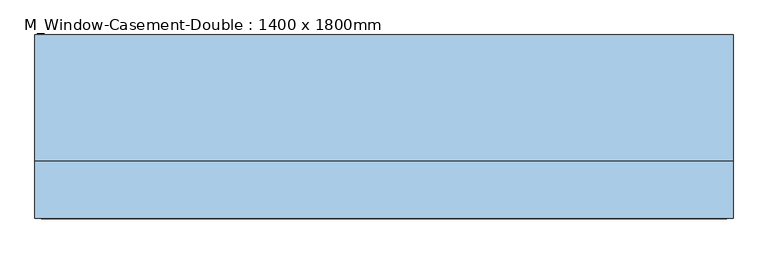
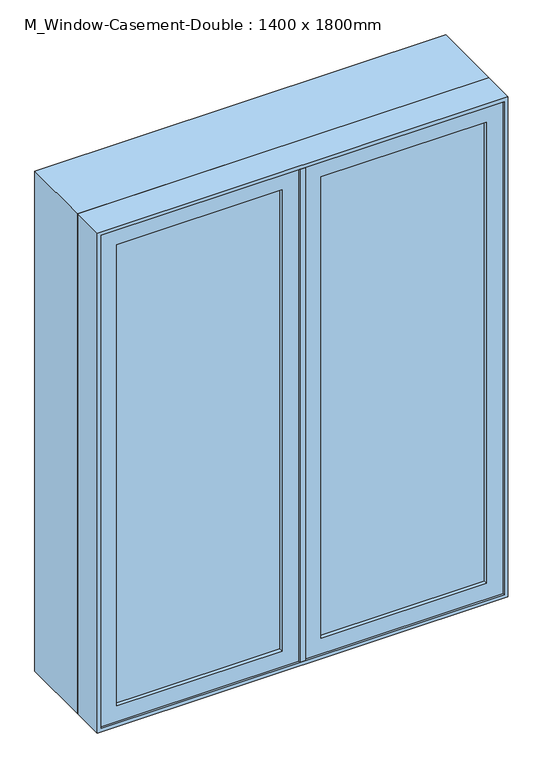
"""IFC4 building model written with IfcOpenShell, lengths in millimetres: window geometry, M_Window-Casement-Double : 1400 x 1800mm."""

import ifcopenshell
import ifcopenshell.guid

model = None  # the IFC model being written
_history = None  # IfcOwnerHistory: only IFC2X3 demands one
_inside = {}  # id of a spatial element -> (the spatial element, [elements in it])
_under = {}  # id of a project, library or spatial element -> (it, [spatial elements below it])
_declared = {}  # id of a project -> (the project, [libraries it declares])
_typed = {}  # id of a type object -> (the type object, [elements of that type])
_made_of = {}  # id of a material, layer set ... -> (it, [elements and type objects made of it])


def new_model(schema):
    """Start an empty IFC model of exactly this schema.

    Asked for "IFC4X3", IfcOpenShell would pick the latest addendum, in which some entities
    have other attributes; the version numbers below select the first issue.
    IFC2X3 requires an IfcOwnerHistory on every rooted entity: one is made here for all.
    """
    global model, _history
    if schema == "IFC4X3":
        model = ifcopenshell.file(schema_version=(4, 3, 0, 0))
    else:
        model = ifcopenshell.file(schema=schema)
    _inside.clear()
    _under.clear()
    _declared.clear()
    _typed.clear()
    _made_of.clear()
    _history = None
    if model.schema == "IFC2X3":
        org = make("IfcOrganization", Name="unknown")
        user = make(
            "IfcPersonAndOrganization",
            ThePerson=make("IfcPerson", FamilyName="unknown"),
            TheOrganization=org,
        )
        app = make(
            "IfcApplication",
            ApplicationDeveloper=org,
            Version="unknown",
            ApplicationFullName="unknown",
            ApplicationIdentifier="unknown",
        )
        _history = make(
            "IfcOwnerHistory",
            OwningUser=user,
            OwningApplication=app,
            ChangeAction="ADDED",
            CreationDate=0,
        )
    return model


def make(cls, **values):
    """One entity of the class cls with the attributes given. An attribute that is None is left unset."""
    return model.create_entity(
        cls, **{name: value for name, value in values.items() if value is not None}
    )


def rooted(cls, **values):
    """An entity with a GlobalId (a new one), such as an element, a storey or a relation."""
    return make(cls, GlobalId=ifcopenshell.guid.new(), OwnerHistory=_history, **values)


def si_unit(unit_type, name, prefix=None):
    """IfcSIUnit, for example si_unit("LENGTHUNIT", "METRE", prefix="MILLI")."""
    return make("IfcSIUnit", UnitType=unit_type, Prefix=prefix, Name=name)


def assignment(units):
    """IfcUnitAssignment: the units of a project."""
    return None if units is None else make("IfcUnitAssignment", Units=units)


def point(xyz):
    """IfcCartesianPoint."""
    return None if xyz is None else make("IfcCartesianPoint", Coordinates=xyz)


def direction(xyz):
    """IfcDirection."""
    return None if xyz is None else make("IfcDirection", DirectionRatios=xyz)


def frame(location, z_axis=None, x_axis=None):
    """IfcAxis2Placement3D, a coordinate frame: its origin and axes. An axis left out is left unset."""
    return make(
        "IfcAxis2Placement3D",
        Location=point(location),
        Axis=direction(z_axis),
        RefDirection=direction(x_axis),
    )


def origin():
    """The frame at (0, 0, 0) with its axes left unset."""
    return frame((0.0, 0.0, 0.0))


def place(relative_to, where):
    """IfcLocalPlacement: puts the frame where relative to a parent placement (None: the world)."""
    return make(
        "IfcLocalPlacement", PlacementRelTo=relative_to, RelativePlacement=where
    )


def context(
    kind, dimensions, precision=None, world=None, true_north=None, identifier=None
):
    """IfcGeometricRepresentationContext, for example the 3D "Model" context."""
    return make(
        "IfcGeometricRepresentationContext",
        ContextIdentifier=identifier,
        ContextType=kind,
        CoordinateSpaceDimension=dimensions,
        Precision=precision,
        WorldCoordinateSystem=world,
        TrueNorth=true_north,
    )


def project(units=None, contexts=None):
    """IfcProject with its units and contexts."""
    return rooted(
        "IfcProject",
        Name="project",
        RepresentationContexts=contexts,
        UnitsInContext=assignment(units),
    )


def spatial(cls, under=None, at=None, **own):
    """A site, building, storey or space (cls), placed at a placement, below another one or the project."""
    s = rooted(cls, ObjectPlacement=at, **own)
    if under is not None:
        _under.setdefault(under.id(), (under, []))[1].append(s)
    return s


def polyline(points):
    """IfcPolyline through the points."""
    return make("IfcPolyline", Points=[point(p) for p in points])


def outline(outer, holes=None, kind="AREA"):
    """IfcArbitraryClosedProfileDef: a profile drawn as a closed curve; with holes, ...WithVoids."""
    if holes is None:
        return make("IfcArbitraryClosedProfileDef", ProfileType=kind, OuterCurve=outer)
    return make(
        "IfcArbitraryProfileDefWithVoids",
        ProfileType=kind,
        OuterCurve=outer,
        InnerCurves=holes,
    )


def extrude(swept, where, along, depth):
    """IfcExtrudedAreaSolid: the profile swept, set in the frame where, extruded along a direction by depth."""
    return make(
        "IfcExtrudedAreaSolid",
        SweptArea=swept,
        Position=where,
        ExtrudedDirection=direction(along),
        Depth=depth,
    )


def faces_of(points, faces, orient=None, outer=None):
    """IfcFace entities. A face is a list of loops; a loop is a list of indices into points, from 0.

    orient and outer hold one flag for each loop. By default every Orientation is true, the
    first loop of a face is its IfcFaceOuterBound and the others are IfcFaceBound.
    """
    made = []
    for i, loops in enumerate(faces):
        bounds = []
        for j, loop in enumerate(loops):
            is_outer = j == 0 if outer is None else outer[i][j]
            bounds.append(
                make(
                    "IfcFaceOuterBound" if is_outer else "IfcFaceBound",
                    Bound=make("IfcPolyLoop", Polygon=[points[k] for k in loop]),
                    Orientation=True if orient is None else orient[i][j],
                )
            )
        made.append(make("IfcFace", Bounds=bounds))
    return made


def faceted_brep(points, faces, orient=None, outer=None, voids=None):
    """IfcFacetedBrep: a solid bounded by flat faces; with voids (closed shells), ...WithVoids."""
    shared = [point(p) for p in points]
    hull = make("IfcClosedShell", CfsFaces=faces_of(shared, faces, orient, outer))
    if voids is None:
        return make("IfcFacetedBrep", Outer=hull)
    return make(
        "IfcFacetedBrepWithVoids",
        Outer=hull,
        Voids=[
            make(cls, CfsFaces=faces_of(shared, fs, o, b)) for cls, fs, o, b in voids
        ],
    )


def shape(context_of_items, identifier, shape_type, items):
    """IfcShapeRepresentation: the items that make up one representation, for example the "Body"."""
    return make(
        "IfcShapeRepresentation",
        ContextOfItems=context_of_items,
        RepresentationIdentifier=identifier,
        RepresentationType=shape_type,
        Items=items,
    )


def source(mapping_origin, context_of_items, identifier, shape_type, items):
    """IfcRepresentationMap: a shape defined once, which mapped items show again and again."""
    return make(
        "IfcRepresentationMap",
        MappingOrigin=mapping_origin,
        MappedRepresentation=shape(context_of_items, identifier, shape_type, items),
    )


def transform(
    local_origin,
    x_axis=None,
    y_axis=None,
    z_axis=None,
    scale=None,
    scale2=None,
    scale3=None,
    uniform=True,
):
    """IfcCartesianTransformationOperator3D, or its non-uniform kind. x_axis, y_axis, z_axis: its Axis1, 2, 3."""
    if uniform:
        return make(
            "IfcCartesianTransformationOperator3D",
            Axis1=direction(x_axis),
            Axis2=direction(y_axis),
            LocalOrigin=point(local_origin),
            Scale=scale,
            Axis3=direction(z_axis),
        )
    return make(
        "IfcCartesianTransformationOperator3DnonUniform",
        Axis1=direction(x_axis),
        Axis2=direction(y_axis),
        LocalOrigin=point(local_origin),
        Scale=scale,
        Axis3=direction(z_axis),
        Scale2=scale2,
        Scale3=scale3,
    )


def mapped(mapping_source, mapping_target):
    """IfcMappedItem: shows the shape of a source again, moved by a transform."""
    return make(
        "IfcMappedItem", MappingSource=mapping_source, MappingTarget=mapping_target
    )


def made_of(thing, what):
    """Note that an element or type object is made of a material, layer set ...; save() writes the relation."""
    if what is not None:
        _made_of.setdefault(what.id(), (what, []))[1].append(thing)
    return thing


def element(
    cls,
    number,
    at=None,
    inside=None,
    cuts=None,
    type_object=None,
    material=None,
    context=None,
    identifier="Body",
    shape_type=None,
    held_by="IfcProductDefinitionShape",
    body=None,
    shapes=None,
    **own,
):
    """One element of the class cls, such as IfcWall. Its Tag is "e" and its number.

    at: its placement. inside: the storey or other place that contains it. cuts: it is an
    opening in that element (IfcRelVoidsElement). A single representation is given by context,
    identifier, shape_type and body (its items); several are given by shapes. held_by: the class
    of the entity that holds the representations. save() writes the other relations.
    """
    e = rooted(cls, Tag="e%d" % number, ObjectPlacement=at, **own)
    if body is not None:
        shapes = [shape(context, identifier, shape_type, body)]
    if shapes is not None:
        e.Representation = make(held_by, Representations=shapes)
    if inside is not None:
        _inside.setdefault(inside.id(), (inside, []))[1].append(e)
    if cuts is not None:
        rooted(
            "IfcRelVoidsElement", RelatingBuildingElement=cuts, RelatedOpeningElement=e
        )
    if type_object is not None:
        _typed.setdefault(type_object.id(), (type_object, []))[1].append(e)
    return made_of(e, material)


def aggregate(whole, parts):
    """IfcRelAggregates: a whole, such as a stair, and the parts it consists of."""
    return rooted("IfcRelAggregates", RelatingObject=whole, RelatedObjects=parts)


def save(model, path):
    """Write the relations noted so far, then the file.

    IfcRelAggregates (storeys below a building ...), IfcRelContainedInSpatialStructure (elements
    in a storey), IfcRelDefinesByType, IfcRelAssociatesMaterial and IfcRelDeclares: one each for
    every whole, place, type object, material and project.
    """
    for whole, parts in _under.values():
        aggregate(whole, parts)
    for where, things in _inside.values():
        rooted(
            "IfcRelContainedInSpatialStructure",
            RelatedElements=things,
            RelatingStructure=where,
        )
    for kind, things in _typed.values():
        rooted("IfcRelDefinesByType", RelatedObjects=things, RelatingType=kind)
    for what, things in _made_of.values():
        rooted("IfcRelAssociatesMaterial", RelatedObjects=things, RelatingMaterial=what)
    for by, libraries in _declared.values():
        rooted("IfcRelDeclares", RelatingContext=by, RelatedDefinitions=libraries)
    model.write(path)


def m_window_casement_double_1400_x_1800mm_42382f28(model_context):
    return source(origin(), model_context, "Body", "SolidModel", [
        faceted_brep([(668.25, -142.75, 2668.25), (-668.25, -142.75, 2668.25), (-668.25, -79.25, 2668.25), (668.25, -79.25, 2668.25), (687.3, -193.55, 2687.3), (-687.3, -193.55, 2687.3), (-687.3, -142.75, 2687.3), (687.3, -142.75, 2687.3), (700.0, -79.25, 2700.0), (-700.0, -79.25, 2700.0), (-700.0, -193.55, 2700.0), (700.0, -193.55, 2700.0), (-668.25, -142.75, 931.75), (-668.25, -79.25, 931.75), (-687.3, -193.55, 912.7), (-687.3, -142.75, 912.7), (-700.0, -79.25, 900.0), (-700.0, -193.55, 900.0), (668.25, -142.75, 931.75), (668.25, -79.25, 931.75), (687.3, -193.55, 912.7), (687.3, -142.75, 912.7), (700.0, -79.25, 900.0), (700.0, -193.55, 900.0)], [[[0, 1, 2, 3]], [[4, 5, 6, 7]], [[8, 9, 10, 11]], [[1, 12, 13, 2]], [[5, 14, 15, 6]], [[9, 16, 17, 10]], [[12, 18, 19, 13]], [[14, 20, 21, 15]], [[16, 22, 23, 17]], [[9, 8, 22, 16], [3, 2, 13, 19]], [[18, 0, 3, 19]], [[7, 6, 15, 21], [1, 0, 18, 12]], [[20, 4, 7, 21]], [[22, 8, 11, 23]], [[11, 10, 17, 23], [5, 4, 20, 14]]]),
        extrude(outline(polyline([(2700.0, -700.0), (900.0, -700.0), (900.0, 700.0), (2700.0, 700.0), (2700.0, -700.0)]), holes=[polyline([(2680.95, 680.95), (919.05, 680.95), (919.05, -680.95), (2680.95, -680.95), (2680.95, 680.95)])]), frame((0.0, -79.25, 0.0), z_axis=(0.0, 1.0, 0.0), x_axis=(0.0, 0.0, 1.0)), (0.0, 0.0, 1.0), 253.75),
        extrude(outline(polyline([(912.7, 9.525), (912.7, 687.3), (2687.3, 687.3), (2687.3, 9.525), (912.7, 9.525)]), holes=[polyline([(969.85, 630.15), (969.85, 66.675), (2630.15, 66.675), (2630.15, 630.15), (969.85, 630.15)])]), frame((0.0, -187.2, 0.0), z_axis=(0.0, 1.0, 0.0), x_axis=(0.0, 0.0, 1.0)), (0.0, 0.0, 1.0), 44.45),
        extrude(outline(polyline([(2687.3, -9.525), (2687.3, -687.3), (912.7, -687.3), (912.7, -9.525), (2687.3, -9.525)]), holes=[polyline([(2630.15, -630.15), (2630.15, -66.675), (969.85, -66.675), (969.85, -630.15), (2630.15, -630.15)])]), frame((0.0, -187.2, 0.0), z_axis=(0.0, 1.0, 0.0), x_axis=(0.0, 0.0, 1.0)), (0.0, 0.0, 1.0), 44.45),
        extrude(outline(polyline([(630.15, -174.5), (66.675, -174.5), (66.675, -168.15), (630.15, -168.15), (630.15, -174.5)])), frame((0.0, 0.0, 969.85), z_axis=(0.0, 0.0, 1.0), x_axis=(1.0, 0.0, 0.0)), (0.0, 0.0, 1.0), 1660.3),
        extrude(outline(polyline([(66.675, -155.45), (630.15, -155.45), (630.15, -161.8), (66.675, -161.8), (66.675, -155.45)])), frame((0.0, 0.0, 969.85), z_axis=(0.0, 0.0, 1.0), x_axis=(1.0, 0.0, 0.0)), (0.0, 0.0, 1.0), 1660.3),
        extrude(outline(polyline([(-66.675, -174.5), (-630.15, -174.5), (-630.15, -168.15), (-66.675, -168.15), (-66.675, -174.5)])), frame((0.0, 0.0, 969.85), z_axis=(0.0, 0.0, 1.0), x_axis=(1.0, 0.0, 0.0)), (0.0, 0.0, 1.0), 1660.3),
        extrude(outline(polyline([(-630.15, -155.45), (-66.675, -155.45), (-66.675, -161.8), (-630.15, -161.8), (-630.15, -155.45)])), frame((0.0, 0.0, 969.85), z_axis=(0.0, 0.0, 1.0), x_axis=(1.0, 0.0, 0.0)), (0.0, 0.0, 1.0), 1660.3),
        faceted_brep([(9.525, -193.55, 2687.3), (9.525, -142.75, 2687.3), (-9.525, -142.75, 2687.3), (-9.525, -193.55, 2687.3), (9.525, -193.55, 912.7), (-9.525, -193.55, 912.7), (-9.525, -142.75, 912.7), (9.525, -142.75, 912.7), (-9.525, -142.75, 2668.25), (-9.525, -142.75, 931.75), (-30.1625, -142.75, 2668.25), (-30.1625, -142.75, 931.75), (-30.1625, -79.25, 2668.25), (-30.1625, -79.25, 931.75), (30.1625, -79.25, 2668.25), (30.1625, -79.25, 931.75), (30.1625, -142.75, 2668.25), (30.1625, -142.75, 931.75), (9.525, -142.75, 2668.25), (9.525, -142.75, 931.75)], [[[0, 1, 2, 3]], [[4, 5, 6, 7]], [[3, 5, 4, 0]], [[2, 8, 9, 6, 5, 3]], [[8, 10, 11, 9]], [[10, 12, 13, 11]], [[12, 14, 15, 13]], [[14, 16, 17, 15]], [[16, 18, 19, 17]], [[0, 4, 7, 19, 18, 1]], [[8, 2, 1, 18]], [[19, 7, 6, 9]], [[9, 11, 13, 15, 17, 19]], [[18, 16, 14, 12, 10, 8]]]),
    ])


if __name__ == "__main__":
    model = new_model("IFC4")
    model_context = context("Model", 3, world=origin())
    ifc_project = project(units=[si_unit("LENGTHUNIT", "METRE", prefix="MILLI")], contexts=[model_context])
    site = spatial("IfcSite", under=ifc_project)
    building = spatial("IfcBuilding", under=site)
    placement = place(None, origin())
    m_window_casement_double_1400_x_1800mm_shape = m_window_casement_double_1400_x_1800mm_42382f28(model_context)
    element("IfcWindow", 1, ObjectType="M_Window-Casement-Double : 1400 x 1800mm", at=placement, inside=building, context=model_context, shape_type="MappedRepresentation", body=[
        mapped(m_window_casement_double_1400_x_1800mm_shape, transform((0.0, 0.0, 0.0), x_axis=(1.0, 0.0, 0.0), y_axis=(0.0, 1.0, 0.0), z_axis=(0.0, 0.0, 1.0))),
    ])
    save(model, "model.ifc")

# Revit data of these elements
# Type "M_Window-Casement-Double : 1400 x 1800mm"
#   Type Mark = "27"
#   Fire Rating = "0.5h"
#   Assembly Code = "B2020100"
#   Analytic Construction = "Double glazing - domestic"
#   Frame Extension [instance default] = 6.35 mm
#   Window Inset [instance default] = 0 mm
#   Wall Thickness [instance default] = 150 mm
#   Interior Wall Closure [instance default] = 54.75 mm
#   Half Width = 700 mm
#   Visual Light Transmittance = 0.81
#   Thermal Resistance (R) = 0.319569 (m²·K)/W
#   Solar Heat Gain Coefficient = 0.76
#   Rough Width = 1415 mm
#   Rough Height = 1815 mm
#   Height = 1800 mm
#   Heat Transfer Coefficient (U) = 3.12929 W/(m²·K)
#   Exterior Wall Closure [instance default] = 31.8 mm
#   Extension Jamb [instance default] = 54.75 mm
#   Default Sill Height = 900 mm
#   Width = 1400 mm
#   Muntin Visibility = yes
#   Interior Trim Visibility [instance default] = yes
#   Exterior Trim Visibility [instance default] = yes
#   Extension Jamb Visibility [instance default] = yes
#   Interior Trim Material = Wood - Stained
#   Muntin Pattern = M_Muntin Pattern_2x2 : M_Muntin Pattern_2x2
#   Interior Trim = M_Trim-Window-Interior-Flat : Picture Frame
#   Interior Frame Material = Wood - Stained
#   Glass Panel Material = Glass
#   Exterior Trim Material = Clad - White
#   Exterior Trim = M_Trim-Window-Exterior-Flat : with Sill
#   Exterior Frame Material = Clad - White
#   Wall Closure = (empty or 0)
# Element 1 (IfcWindow, "M_Window-Casement-Double : 1400 x 1800mm")
#   Wall Thickness = 349 mm
#   Extension Jamb = 253.75 mm
#   Materials on its faces: "Wood - Stained", "Glass", "Clad - White"
# Materials
#   "Wood - Stained": class "Wood", colour RGB 173 132 96, transparency 0, Cost = 0
#   "Glass": class "Glass", colour RGB 245 245 243, transparency 1, Description = "Soda Lime Glass", Cost = 0
#   "Clad - White": class "Wood", colour RGB 245 245 243, transparency 0, Cost = 0
